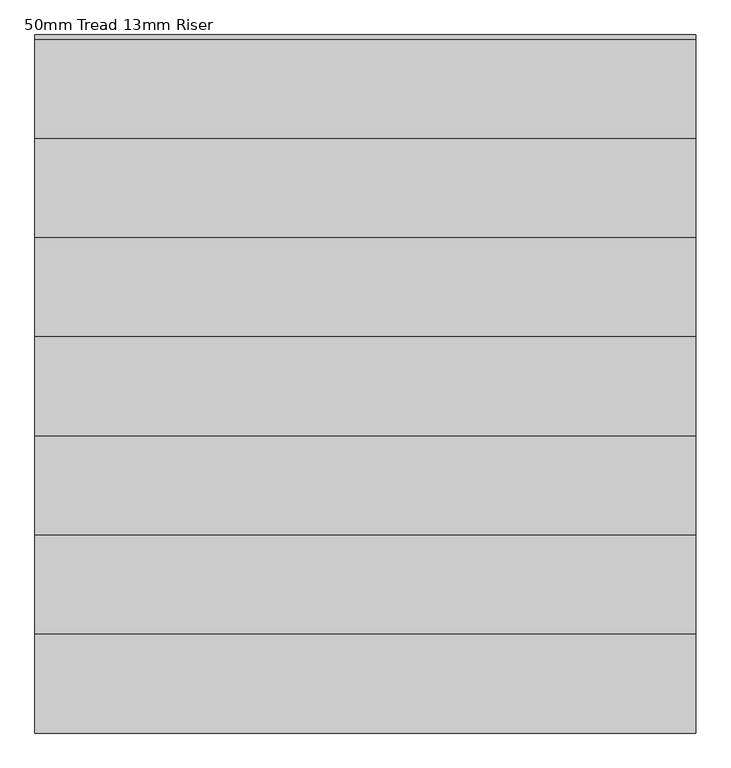
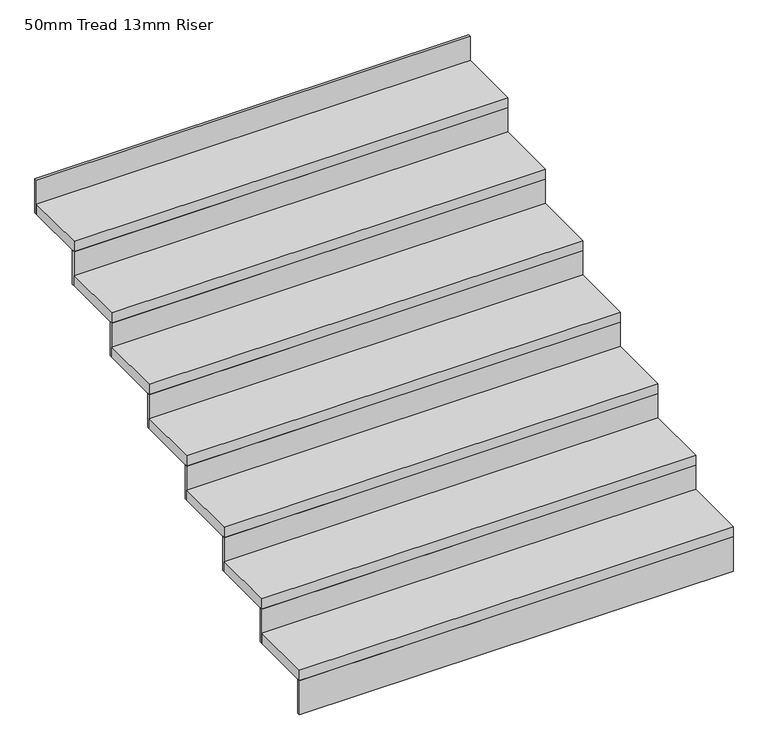
"""IFC4 building model written with IfcOpenShell, lengths in millimetres: stair flight geometry, 50mm Tread 13mm Riser."""

from ifc_helpers import new_model, si_unit, frame, origin, place, context, project, spatial, polyline, outline, extrude, source, transform, mapped, element, save


def stair_flight_50mm_tread_13mm_riser_3c25b415(model_context):
    return source(origin(), model_context, "Body", "SweptSolid", [
        extrude(outline(polyline([(14700.0002443, 21382.4999999), (14700.0002443, 21369.9999999), (12700.0002443, 21369.9999999), (12700.0002443, 21382.4999999), (14700.0002443, 21382.4999999)])), frame((0.0, 0.0, 29116.6666667), z_axis=(0.0, 0.0, 1.0), x_axis=(1.0, 0.0, 0.0)), (0.0, 0.0, 1.0), 166.6666667),
        extrude(outline(polyline([(12700.0002443, 21669.9999999), (14700.0002443, 21669.9999999), (14700.0002443, 21369.9999999), (12700.0002443, 21369.9999999), (12700.0002443, 21669.9999999)])), frame((0.0, 0.0, 29283.3333333), z_axis=(0.0, 0.0, 1.0), x_axis=(1.0, 0.0, 0.0)), (0.0, 0.0, 1.0), 50.0),
        extrude(outline(polyline([(14700.0002443, 21682.4999999), (14700.0002443, 21669.9999999), (12700.0002443, 21669.9999999), (12700.0002443, 21682.4999999), (14700.0002443, 21682.4999999)])), frame((0.0, 0.0, 29283.3333333), z_axis=(0.0, 0.0, 1.0), x_axis=(1.0, 0.0, 0.0)), (0.0, 0.0, 1.0), 166.6666667),
        extrude(outline(polyline([(12700.0002443, 21969.9999999), (14700.0002443, 21969.9999999), (14700.0002443, 21669.9999999), (12700.0002443, 21669.9999999), (12700.0002443, 21969.9999999)])), frame((0.0, 0.0, 29450.0), z_axis=(0.0, 0.0, 1.0), x_axis=(1.0, 0.0, 0.0)), (0.0, 0.0, 1.0), 50.0),
        extrude(outline(polyline([(14700.0002443, 21982.4999999), (14700.0002443, 21969.9999999), (12700.0002443, 21969.9999999), (12700.0002443, 21982.4999999), (14700.0002443, 21982.4999999)])), frame((0.0, 0.0, 29450.0), z_axis=(0.0, 0.0, 1.0), x_axis=(1.0, 0.0, 0.0)), (0.0, 0.0, 1.0), 166.6666667),
        extrude(outline(polyline([(12700.0002443, 22269.9999999), (14700.0002443, 22269.9999999), (14700.0002443, 21969.9999999), (12700.0002443, 21969.9999999), (12700.0002443, 22269.9999999)])), frame((0.0, 0.0, 29616.6666667), z_axis=(0.0, 0.0, 1.0), x_axis=(1.0, 0.0, 0.0)), (0.0, 0.0, 1.0), 50.0),
        extrude(outline(polyline([(14700.0002443, 22282.4999999), (14700.0002443, 22269.9999999), (12700.0002443, 22269.9999999), (12700.0002443, 22282.4999999), (14700.0002443, 22282.4999999)])), frame((0.0, 0.0, 29616.6666667), z_axis=(0.0, 0.0, 1.0), x_axis=(1.0, 0.0, 0.0)), (0.0, 0.0, 1.0), 166.6666667),
        extrude(outline(polyline([(12700.0002443, 22569.9999999), (14700.0002443, 22569.9999999), (14700.0002443, 22269.9999999), (12700.0002443, 22269.9999999), (12700.0002443, 22569.9999999)])), frame((0.0, 0.0, 29783.3333333), z_axis=(0.0, 0.0, 1.0), x_axis=(1.0, 0.0, 0.0)), (0.0, 0.0, 1.0), 50.0),
        extrude(outline(polyline([(14700.0002443, 22582.4999999), (14700.0002443, 22569.9999999), (12700.0002443, 22569.9999999), (12700.0002443, 22582.4999999), (14700.0002443, 22582.4999999)])), frame((0.0, 0.0, 29783.3333333), z_axis=(0.0, 0.0, 1.0), x_axis=(1.0, 0.0, 0.0)), (0.0, 0.0, 1.0), 166.6666667),
        extrude(outline(polyline([(12700.0002443, 22869.9999999), (14700.0002443, 22869.9999999), (14700.0002443, 22569.9999999), (12700.0002443, 22569.9999999), (12700.0002443, 22869.9999999)])), frame((0.0, 0.0, 29950.0), z_axis=(0.0, 0.0, 1.0), x_axis=(1.0, 0.0, 0.0)), (0.0, 0.0, 1.0), 50.0),
        extrude(outline(polyline([(14700.0002443, 22882.4999999), (14700.0002443, 22869.9999999), (12700.0002443, 22869.9999999), (12700.0002443, 22882.4999999), (14700.0002443, 22882.4999999)])), frame((0.0, 0.0, 29950.0), z_axis=(0.0, 0.0, 1.0), x_axis=(1.0, 0.0, 0.0)), (0.0, 0.0, 1.0), 166.6666667),
        extrude(outline(polyline([(12700.0002443, 23169.9999999), (14700.0002443, 23169.9999999), (14700.0002443, 22869.9999999), (12700.0002443, 22869.9999999), (12700.0002443, 23169.9999999)])), frame((0.0, 0.0, 30116.6666667), z_axis=(0.0, 0.0, 1.0), x_axis=(1.0, 0.0, 0.0)), (0.0, 0.0, 1.0), 50.0),
        extrude(outline(polyline([(14700.0002443, 23182.4999999), (14700.0002443, 23169.9999999), (12700.0002443, 23169.9999999), (12700.0002443, 23182.4999999), (14700.0002443, 23182.4999999)])), frame((0.0, 0.0, 30116.6666667), z_axis=(0.0, 0.0, 1.0), x_axis=(1.0, 0.0, 0.0)), (0.0, 0.0, 1.0), 166.6666667),
        extrude(outline(polyline([(14700.0002443, 23482.4999999), (14700.0002443, 23469.9999999), (12700.0002443, 23469.9999999), (12700.0002443, 23482.4999999), (14700.0002443, 23482.4999999)])), frame((0.0, 0.0, 30283.3333333), z_axis=(0.0, 0.0, 1.0), x_axis=(1.0, 0.0, 0.0)), (0.0, 0.0, 1.0), 166.6666667),
        extrude(outline(polyline([(12700.0002443, 23469.9999999), (14700.0002443, 23469.9999999), (14700.0002443, 23169.9999999), (12700.0002443, 23169.9999999), (12700.0002443, 23469.9999999)])), frame((0.0, 0.0, 30283.3333333), z_axis=(0.0, 0.0, 1.0), x_axis=(1.0, 0.0, 0.0)), (0.0, 0.0, 1.0), 50.0),
    ])


if __name__ == "__main__":
    model = new_model("IFC4")
    model_context = context("Model", 3, world=origin())
    ifc_project = project(units=[si_unit("LENGTHUNIT", "METRE", prefix="MILLI")], contexts=[model_context])
    site = spatial("IfcSite", under=ifc_project)
    building = spatial("IfcBuilding", under=site)
    placement = place(None, origin())
    stair_flight_50mm_tread_13mm_riser_shape = stair_flight_50mm_tread_13mm_riser_3c25b415(model_context)
    element("IfcStairFlight", 1, ObjectType="50mm Tread 13mm Riser", at=placement, inside=building, context=model_context, shape_type="MappedRepresentation", body=[
        mapped(stair_flight_50mm_tread_13mm_riser_shape, transform((0.0, 0.0, 0.0), x_axis=(1.0, 0.0, 0.0), y_axis=(0.0, 1.0, 0.0), z_axis=(0.0, 0.0, 1.0))),
    ])
    save(model, "model.ifc")
